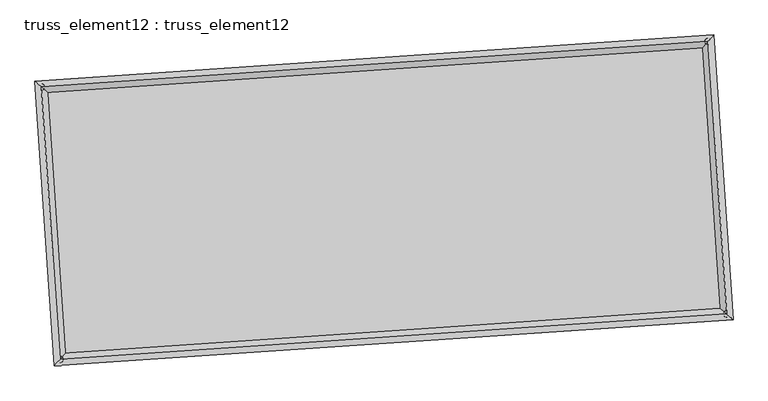
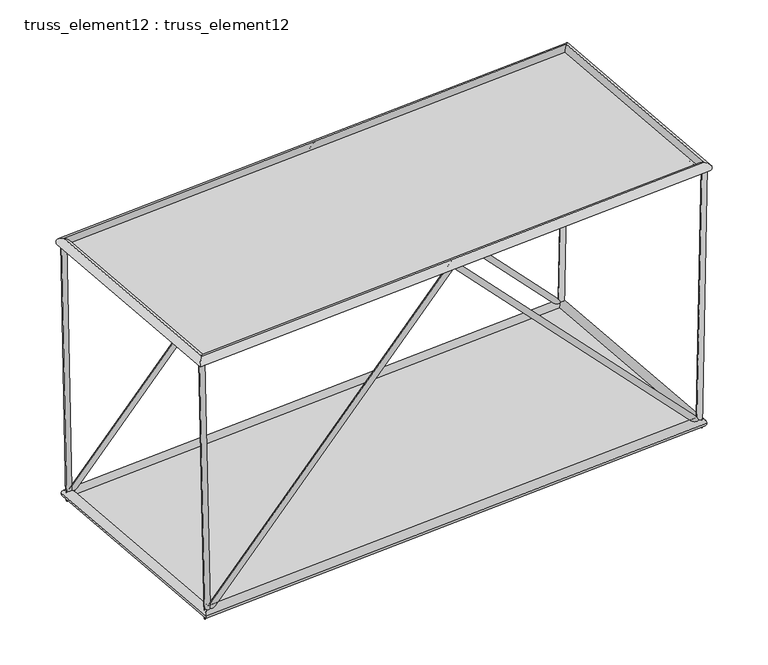
"""IFC4 building model written with IfcOpenShell, lengths in millimetres: plate geometry, truss_element12 : truss_element12."""

import ifcopenshell
import ifcopenshell.guid

model = None  # the IFC model being written
_history = None  # IfcOwnerHistory: only IFC2X3 demands one
_inside = {}  # id of a spatial element -> (the spatial element, [elements in it])
_under = {}  # id of a project, library or spatial element -> (it, [spatial elements below it])
_declared = {}  # id of a project -> (the project, [libraries it declares])
_typed = {}  # id of a type object -> (the type object, [elements of that type])
_made_of = {}  # id of a material, layer set ... -> (it, [elements and type objects made of it])


def new_model(schema):
    """Start an empty IFC model of exactly this schema.

    Asked for "IFC4X3", IfcOpenShell would pick the latest addendum, in which some entities
    have other attributes; the version numbers below select the first issue.
    IFC2X3 requires an IfcOwnerHistory on every rooted entity: one is made here for all.
    """
    global model, _history
    if schema == "IFC4X3":
        model = ifcopenshell.file(schema_version=(4, 3, 0, 0))
    else:
        model = ifcopenshell.file(schema=schema)
    _inside.clear()
    _under.clear()
    _declared.clear()
    _typed.clear()
    _made_of.clear()
    _history = None
    if model.schema == "IFC2X3":
        org = make("IfcOrganization", Name="unknown")
        user = make(
            "IfcPersonAndOrganization",
            ThePerson=make("IfcPerson", FamilyName="unknown"),
            TheOrganization=org,
        )
        app = make(
            "IfcApplication",
            ApplicationDeveloper=org,
            Version="unknown",
            ApplicationFullName="unknown",
            ApplicationIdentifier="unknown",
        )
        _history = make(
            "IfcOwnerHistory",
            OwningUser=user,
            OwningApplication=app,
            ChangeAction="ADDED",
            CreationDate=0,
        )
    return model


def make(cls, **values):
    """One entity of the class cls with the attributes given. An attribute that is None is left unset."""
    return model.create_entity(
        cls, **{name: value for name, value in values.items() if value is not None}
    )


def rooted(cls, **values):
    """An entity with a GlobalId (a new one), such as an element, a storey or a relation."""
    return make(cls, GlobalId=ifcopenshell.guid.new(), OwnerHistory=_history, **values)


def si_unit(unit_type, name, prefix=None):
    """IfcSIUnit, for example si_unit("LENGTHUNIT", "METRE", prefix="MILLI")."""
    return make("IfcSIUnit", UnitType=unit_type, Prefix=prefix, Name=name)


def assignment(units):
    """IfcUnitAssignment: the units of a project."""
    return None if units is None else make("IfcUnitAssignment", Units=units)


def point(xyz):
    """IfcCartesianPoint."""
    return None if xyz is None else make("IfcCartesianPoint", Coordinates=xyz)


def direction(xyz):
    """IfcDirection."""
    return None if xyz is None else make("IfcDirection", DirectionRatios=xyz)


def frame(location, z_axis=None, x_axis=None):
    """IfcAxis2Placement3D, a coordinate frame: its origin and axes. An axis left out is left unset."""
    return make(
        "IfcAxis2Placement3D",
        Location=point(location),
        Axis=direction(z_axis),
        RefDirection=direction(x_axis),
    )


def origin():
    """The frame at (0, 0, 0) with its axes left unset."""
    return frame((0.0, 0.0, 0.0))


def origin_with_axes():
    """The frame at (0, 0, 0) with the z axis (0, 0, 1) and the x axis (1, 0, 0) written out."""
    return frame((0.0, 0.0, 0.0), z_axis=(0.0, 0.0, 1.0), x_axis=(1.0, 0.0, 0.0))


def place(relative_to, where):
    """IfcLocalPlacement: puts the frame where relative to a parent placement (None: the world)."""
    return make(
        "IfcLocalPlacement", PlacementRelTo=relative_to, RelativePlacement=where
    )


def context(
    kind, dimensions, precision=None, world=None, true_north=None, identifier=None
):
    """IfcGeometricRepresentationContext, for example the 3D "Model" context."""
    return make(
        "IfcGeometricRepresentationContext",
        ContextIdentifier=identifier,
        ContextType=kind,
        CoordinateSpaceDimension=dimensions,
        Precision=precision,
        WorldCoordinateSystem=world,
        TrueNorth=true_north,
    )


def project(units=None, contexts=None):
    """IfcProject with its units and contexts."""
    return rooted(
        "IfcProject",
        Name="project",
        RepresentationContexts=contexts,
        UnitsInContext=assignment(units),
    )


def spatial(cls, under=None, at=None, **own):
    """A site, building, storey or space (cls), placed at a placement, below another one or the project."""
    s = rooted(cls, ObjectPlacement=at, **own)
    if under is not None:
        _under.setdefault(under.id(), (under, []))[1].append(s)
    return s


def polyline(points):
    """IfcPolyline through the points."""
    return make("IfcPolyline", Points=[point(p) for p in points])


def circle_curve(where, radius):
    """IfcCircle in the frame where."""
    return make("IfcCircle", Position=where, Radius=radius)


def ellipse_curve(where, semi_axis1, semi_axis2):
    """IfcEllipse in the frame where."""
    return make(
        "IfcEllipse", Position=where, SemiAxis1=semi_axis1, SemiAxis2=semi_axis2
    )


def outline(outer, holes=None, kind="AREA"):
    """IfcArbitraryClosedProfileDef: a profile drawn as a closed curve; with holes, ...WithVoids."""
    if holes is None:
        return make("IfcArbitraryClosedProfileDef", ProfileType=kind, OuterCurve=outer)
    return make(
        "IfcArbitraryProfileDefWithVoids",
        ProfileType=kind,
        OuterCurve=outer,
        InnerCurves=holes,
    )


def extrude(swept, where, along, depth):
    """IfcExtrudedAreaSolid: the profile swept, set in the frame where, extruded along a direction by depth."""
    return make(
        "IfcExtrudedAreaSolid",
        SweptArea=swept,
        Position=where,
        ExtrudedDirection=direction(along),
        Depth=depth,
    )


def shape(context_of_items, identifier, shape_type, items):
    """IfcShapeRepresentation: the items that make up one representation, for example the "Body"."""
    return make(
        "IfcShapeRepresentation",
        ContextOfItems=context_of_items,
        RepresentationIdentifier=identifier,
        RepresentationType=shape_type,
        Items=items,
    )


def source(mapping_origin, context_of_items, identifier, shape_type, items):
    """IfcRepresentationMap: a shape defined once, which mapped items show again and again."""
    return make(
        "IfcRepresentationMap",
        MappingOrigin=mapping_origin,
        MappedRepresentation=shape(context_of_items, identifier, shape_type, items),
    )


def transform(
    local_origin,
    x_axis=None,
    y_axis=None,
    z_axis=None,
    scale=None,
    scale2=None,
    scale3=None,
    uniform=True,
):
    """IfcCartesianTransformationOperator3D, or its non-uniform kind. x_axis, y_axis, z_axis: its Axis1, 2, 3."""
    if uniform:
        return make(
            "IfcCartesianTransformationOperator3D",
            Axis1=direction(x_axis),
            Axis2=direction(y_axis),
            LocalOrigin=point(local_origin),
            Scale=scale,
            Axis3=direction(z_axis),
        )
    return make(
        "IfcCartesianTransformationOperator3DnonUniform",
        Axis1=direction(x_axis),
        Axis2=direction(y_axis),
        LocalOrigin=point(local_origin),
        Scale=scale,
        Axis3=direction(z_axis),
        Scale2=scale2,
        Scale3=scale3,
    )


def mapped(mapping_source, mapping_target):
    """IfcMappedItem: shows the shape of a source again, moved by a transform."""
    return make(
        "IfcMappedItem", MappingSource=mapping_source, MappingTarget=mapping_target
    )


def made_of(thing, what):
    """Note that an element or type object is made of a material, layer set ...; save() writes the relation."""
    if what is not None:
        _made_of.setdefault(what.id(), (what, []))[1].append(thing)
    return thing


def element(
    cls,
    number,
    at=None,
    inside=None,
    cuts=None,
    type_object=None,
    material=None,
    context=None,
    identifier="Body",
    shape_type=None,
    held_by="IfcProductDefinitionShape",
    body=None,
    shapes=None,
    **own,
):
    """One element of the class cls, such as IfcWall. Its Tag is "e" and its number.

    at: its placement. inside: the storey or other place that contains it. cuts: it is an
    opening in that element (IfcRelVoidsElement). A single representation is given by context,
    identifier, shape_type and body (its items); several are given by shapes. held_by: the class
    of the entity that holds the representations. save() writes the other relations.
    """
    e = rooted(cls, Tag="e%d" % number, ObjectPlacement=at, **own)
    if body is not None:
        shapes = [shape(context, identifier, shape_type, body)]
    if shapes is not None:
        e.Representation = make(held_by, Representations=shapes)
    if inside is not None:
        _inside.setdefault(inside.id(), (inside, []))[1].append(e)
    if cuts is not None:
        rooted(
            "IfcRelVoidsElement", RelatingBuildingElement=cuts, RelatedOpeningElement=e
        )
    if type_object is not None:
        _typed.setdefault(type_object.id(), (type_object, []))[1].append(e)
    return made_of(e, material)


def aggregate(whole, parts):
    """IfcRelAggregates: a whole, such as a stair, and the parts it consists of."""
    return rooted("IfcRelAggregates", RelatingObject=whole, RelatedObjects=parts)


def save(model, path):
    """Write the relations noted so far, then the file.

    IfcRelAggregates (storeys below a building ...), IfcRelContainedInSpatialStructure (elements
    in a storey), IfcRelDefinesByType, IfcRelAssociatesMaterial and IfcRelDeclares: one each for
    every whole, place, type object, material and project.
    """
    for whole, parts in _under.values():
        aggregate(whole, parts)
    for where, things in _inside.values():
        rooted(
            "IfcRelContainedInSpatialStructure",
            RelatedElements=things,
            RelatingStructure=where,
        )
    for kind, things in _typed.values():
        rooted("IfcRelDefinesByType", RelatedObjects=things, RelatingType=kind)
    for what, things in _made_of.values():
        rooted("IfcRelAssociatesMaterial", RelatedObjects=things, RelatingMaterial=what)
    for by, libraries in _declared.values():
        rooted("IfcRelDeclares", RelatingContext=by, RelatedDefinitions=libraries)
    model.write(path)


def plane_surface(at):
    """IfcPlane: the flat surface through the origin of the frame at, square to its z axis."""
    return make("IfcPlane", Position=at)


def cylinder_surface(at, radius):
    """IfcCylindricalSurface: all points at the distance radius from the z axis of the frame at."""
    return make("IfcCylindricalSurface", Position=at, Radius=radius)


def advanced_brep(points, edges, surfaces, faces):
    """IfcAdvancedBrep: a solid bounded by faces that lie on surfaces and meet in shared edges.

    An edge is (start, end): straight between two places in points (the first is 0);
    or (start, end, curve); or (start, end, curve, False) where it runs against its curve.
    A face is (place in surfaces, loops), or (place, loops, False) where it looks against
    its surface's normal. A loop lists edges by number (the first is 1), with a minus sign
    where the edge is run from its end to its start. The first loop is the outer one.
    """
    corners = [point(p) for p in points]
    vertices = [make("IfcVertexPoint", VertexGeometry=c) for c in corners]
    made = []
    for start, end, *more in edges:
        made.append(
            make(
                "IfcEdgeCurve",
                EdgeStart=vertices[start],
                EdgeEnd=vertices[end],
                EdgeGeometry=more[0] if more else make("IfcPolyline", Points=[corners[start], corners[end]]),
                SameSense=more[1] if len(more) > 1 else True,
            )
        )
    hull = []
    for where, loops, *sense in faces:
        bounds = []
        for j, loop in enumerate(loops):
            ring = [make("IfcOrientedEdge", EdgeElement=made[abs(k) - 1], Orientation=k > 0) for k in loop]
            bounds.append(
                make(
                    "IfcFaceOuterBound" if j == 0 else "IfcFaceBound",
                    Bound=make("IfcEdgeLoop", EdgeList=ring),
                    Orientation=True,
                )
            )
        hull.append(make("IfcAdvancedFace", Bounds=bounds, FaceSurface=surfaces[where], SameSense=sense[0] if sense else True))
    return make("IfcAdvancedBrep", Outer=make("IfcClosedShell", CfsFaces=hull))


def truss_element12_truss_element12_b131e6b3(model_context):
    return source(origin(), model_context, "Body", "SolidModel", [
        advanced_brep(
        [(-3768.4426764, 2269.1666348, 4999.9589336), (-3867.5246147, 2255.8068381, 4997.8888311), (-3667.4480193, 2276.0530765, 121.5783447), (-3761.5388635, 2263.0336036, -121.5783447), (1063.0770133, 2598.6095961, 5071.0530229), (1063.5348076, 2592.0370354, 4926.8211016), (5794.8562778, 2921.251637, 121.5871066), (5889.9046992, 2921.1288515, -121.5871066), (5894.6060324, 2928.0531935, 4999.9725392), (5994.5849006, 2928.2665965, 4997.9279449)],
        [
            (0, 1, circle_curve(frame((-3817.9836456, 2262.4867364, 4998.9238824), z_axis=(-0.02069804082979307, -0.0014113207235644356, 0.9997847764792298), x_axis=(-0.1335984293387775, 0.9910346065567788, -0.0013668522459998886)), 50.0)),
            (1, 0, circle_curve(frame((-3817.9836456, 2262.4867364, 4998.9238824), z_axis=(-0.02069804082979307, -0.0014113207235644356, 0.9997847764792298), x_axis=(-0.1335984293387775, 0.9910346065567788, -0.0013668522459998886)), 50.0)),
            (0, 2),
            (2, 3, ellipse_curve(frame((-3714.4934414, 2269.54334, 0.0), z_axis=(-0.9295901312719013, -0.06338521734851928, 0.3631039824397008), x_axis=(0.3622628143287531, 0.024701324219198188, 0.9317486237910038)), 130.7681897, 50.0)),
            (3, 1),
            (3, 2, ellipse_curve(frame((-3714.4934414, 2269.54334, 0.0), z_axis=(-0.9295901312719013, -0.06338521734851928, 0.3631039824397008), x_axis=(0.3622628143287531, 0.024701324219198188, 0.9317486237910038)), 130.7681897, 50.0)),
            (2, 4),
            (4, 5, ellipse_curve(frame((1063.3059105, 2595.3233157, 4998.9370622), z_axis=(-0.9976833938584647, -0.06802823807757281, -6.665670624892205e-05), x_axis=(6.650228906150557e-05, 4.534538292236935e-06, -0.9999999977784416)), 72.2729929, 50.0)),
            (5, 3),
            (5, 4, ellipse_curve(frame((1063.3059105, 2595.3233157, 4998.9370622), z_axis=(-0.9976833938584647, -0.06802823807757281, -6.665670624892205e-05), x_axis=(6.650228906150557e-05, 4.534538292236935e-06, -0.9999999977784416)), 72.2729929, 50.0)),
            (4, 6),
            (6, 7, ellipse_curve(frame((5842.3804885, 2921.1902443, 0.0), z_axis=(-0.9295196526265941, -0.06338041167761001, -0.3632852031070254), x_axis=(-0.3624436151795683, -0.024713652341926975, 0.9316779814954775)), 130.7875297, 50.0)),
            (7, 5),
            (7, 6, ellipse_curve(frame((5842.3804885, 2921.1902443, 0.0), z_axis=(-0.9295196526265941, -0.06338041167761001, -0.3632852031070254), x_axis=(-0.3624436151795683, -0.024713652341926975, 0.9316779814954775)), 130.7875297, 50.0)),
            (8, 9, circle_curve(frame((5944.5954665, 2928.159895, 4998.950242), z_axis=(0.02044299559371984, 0.0013939301584341597, 0.9997900484050983), x_axis=(-0.0021620821975439704, 0.9999967514320084, -0.001350009629994563)), 50.0)),
            (9, 8, circle_curve(frame((5944.5954665, 2928.159895, 4998.950242), z_axis=(0.02044299559371984, 0.0013939301584341597, 0.9997900484050983), x_axis=(-0.0021620821975439704, 0.9999967514320084, -0.001350009629994563)), 50.0)),
            (6, 8),
            (9, 7),
        ],
        [
            plane_surface(frame((-3817.9836456, 2312.4866866, 4998.9944636), z_axis=(-0.02069804082979222, -0.0014113207235603269, 0.9997847764792298), x_axis=(0.999785772606216, -2.9217833220407372e-05, 0.020698020207497326))),
            cylinder_surface(frame((-3817.9836456, 2262.4867364, 4998.9238824), z_axis=(-0.02069804082979307, -0.0014113207235644356, 0.9997847764792298), x_axis=(-0.1335984293387775, 0.9910346065567788, -0.0013668522459998886)), 50.0),
            cylinder_surface(frame((-3714.4934414, 2269.54334, 0.0), z_axis=(-0.6901706602776504, -0.047060113740035145, -0.7221148145459193), x_axis=(-0.02041427160093359, 0.9987522040196589, -0.04557732419610876)), 50.0),
            cylinder_surface(frame((1063.3059105, 2595.3233157, 4998.9370622), z_axis=(-0.6902666987206849, -0.04706666223638937, 0.7220225854799648), x_axis=(-0.11534052405583756, 0.9922795437132268, -0.04558366635972915)), 50.0),
            plane_surface(frame((5944.5954665, 2878.1599436, 4999.0199531), z_axis=(0.020442995593722254, 0.0013939301584386188, 0.9997900484050981), x_axis=(0.9997910201292843, -2.850206444371398e-05, -0.020442975724616754))),
            cylinder_surface(frame((5842.3804885, 2921.1902443, 0.0), z_axis=(-0.020442995593719836, -0.0013939301584341595, -0.9997900484050981), x_axis=(-0.0021620821975439704, 0.9999967514320084, -0.001350009629994563)), 50.0),
        ],
        [
            (0, [[1, 2]]),
            (1, [[-1, 3, 4, 5]]),
            (1, [[-2, -5, 6, -3]]),
            (2, [[-4, 7, 8, 9]]),
            (2, [[-6, -9, 10, -7]]),
            (3, [[-8, 11, 12, 13]]),
            (3, [[-10, -13, 14, -11]]),
            (4, [[15, 16]]),
            (5, [[-12, 17, -16, 18]]),
            (5, [[-14, -18, -15, -17]]),
        ],
    ),
        advanced_brep(
        [(-3496.3297235, -1721.5669495, 4999.9589336), (-3595.4116618, -1734.9267462, 4997.8888311), (-3395.3350664, -1714.6805078, 121.5783447), (-3489.4259106, -1727.6999807, -121.5783447), (1335.1899662, -1392.1239882, 5071.0530229), (1335.6477605, -1398.6965489, 4926.8211016), (6066.9692307, -1069.4819473, 121.5871066), (6162.0176521, -1069.6047328, -121.5871066), (6166.7189853, -1062.6803908, 4999.9725392), (6266.6978535, -1062.4669878, 4997.9279449)],
        [
            (0, 1, circle_curve(frame((-3545.8706927, -1728.2468479, 4998.9238824), z_axis=(-0.02069804082979312, -0.001411320723564435, 0.9997847764792299), x_axis=(-0.1335984293387778, 0.9910346065567789, -0.001366852245999902)), 50.0)),
            (1, 0, circle_curve(frame((-3545.8706927, -1728.2468479, 4998.9238824), z_axis=(-0.02069804082979312, -0.001411320723564435, 0.9997847764792299), x_axis=(-0.1335984293387778, 0.9910346065567789, -0.001366852245999902)), 50.0)),
            (0, 2),
            (2, 3, ellipse_curve(frame((-3442.3804885, -1721.1902443, 0.0), z_axis=(-0.929590131271901, -0.06338521734851939, 0.36310398243970093), x_axis=(0.36226281432875324, 0.024701324219198247, 0.9317486237910038)), 130.7681897, 50.0)),
            (3, 1),
            (3, 2, ellipse_curve(frame((-3442.3804885, -1721.1902443, 0.0), z_axis=(-0.929590131271901, -0.06338521734851939, 0.36310398243970093), x_axis=(0.36226281432875324, 0.024701324219198247, 0.9317486237910038)), 130.7681897, 50.0)),
            (2, 4),
            (4, 5, ellipse_curve(frame((1335.4188634, -1395.4102686, 4998.9370622), z_axis=(-0.9976833938584647, -0.06802823807757304, -6.665670624852088e-05), x_axis=(6.650228906104429e-05, 4.5345382922849825e-06, -0.9999999977784416)), 72.2729929, 50.0)),
            (5, 3),
            (5, 4, ellipse_curve(frame((1335.4188634, -1395.4102686, 4998.9370622), z_axis=(-0.9976833938584647, -0.06802823807757304, -6.665670624852088e-05), x_axis=(6.650228906104429e-05, 4.5345382922849825e-06, -0.9999999977784416)), 72.2729929, 50.0)),
            (4, 6),
            (6, 7, ellipse_curve(frame((6114.4934414, -1069.54334, 0.0), z_axis=(-0.9295196526265943, -0.06338041167761027, -0.3632852031070244), x_axis=(-0.3624436151795674, -0.02471365234192704, 0.9316779814954779)), 130.7875297, 50.0)),
            (7, 5),
            (7, 6, ellipse_curve(frame((6114.4934414, -1069.54334, 0.0), z_axis=(-0.9295196526265943, -0.06338041167761027, -0.3632852031070244), x_axis=(-0.3624436151795674, -0.02471365234192704, 0.9316779814954779)), 130.7875297, 50.0)),
            (8, 9, circle_curve(frame((6216.7084194, -1062.5736893, 4998.950242), z_axis=(0.020442995593720842, 0.0013939301584342109, 0.9997900484050981), x_axis=(-0.002162082197543998, 0.9999967514320084, -0.0013500096299946115)), 50.0)),
            (9, 8, circle_curve(frame((6216.7084194, -1062.5736893, 4998.950242), z_axis=(0.020442995593720842, 0.0013939301584342109, 0.9997900484050981), x_axis=(-0.002162082197543998, 0.9999967514320084, -0.0013500096299946115)), 50.0)),
            (6, 8),
            (9, 7),
        ],
        [
            plane_surface(frame((-3545.8706927, -1678.2468977, 4998.9944636), z_axis=(-0.020698040829792222, -0.0014113207235603234, 0.9997847764792299), x_axis=(0.999785772606216, -2.9217833220407372e-05, 0.020698020207497326))),
            cylinder_surface(frame((-3545.8706927, -1728.2468479, 4998.9238824), z_axis=(-0.020698040829793124, -0.0014113207235644351, 0.9997847764792301), x_axis=(-0.1335984293387778, 0.9910346065567789, -0.001366852245999902)), 50.0),
            cylinder_surface(frame((-3442.3804885, -1721.1902443, 0.0), z_axis=(-0.6901706602776506, -0.047060113740035256, -0.7221148145459192), x_axis=(-0.020414271600933634, 0.9987522040196589, -0.04557732419610887)), 50.0),
            cylinder_surface(frame((1335.4188634, -1395.4102686, 4998.9370622), z_axis=(-0.6902666987206844, -0.04706666223638954, 0.7220225854799652), x_axis=(-0.115340524055838, 0.9922795437132268, -0.0455836663597292)), 50.0),
            plane_surface(frame((6216.7084194, -1112.5736407, 4999.0199531), z_axis=(0.020442995593722254, 0.0013939301584386132, 0.9997900484050981), x_axis=(0.9997910201292843, -2.8502064444602157e-05, -0.020442975724616754))),
            cylinder_surface(frame((6114.4934414, -1069.54334, 0.0), z_axis=(-0.020442995593720842, -0.0013939301584342109, -0.9997900484050981), x_axis=(-0.002162082197543998, 0.9999967514320084, -0.0013500096299946115)), 50.0),
        ],
        [
            (0, [[1, 2]]),
            (1, [[-1, 3, 4, 5]]),
            (1, [[-2, -5, 6, -3]]),
            (2, [[-4, 7, 8, 9]]),
            (2, [[-6, -9, 10, -7]]),
            (3, [[-8, 11, 12, 13]]),
            (3, [[-10, -13, 14, -11]]),
            (4, [[15, 16]]),
            (5, [[-12, 17, -16, 18]]),
            (5, [[-14, -18, -15, -17]]),
        ],
    ),
        advanced_brep(
        [(-3545.8638321, -1728.2392441, 4908.9238827), (-3545.8775532, -1728.2544517, 5088.9238821), (-3817.9914747, 2262.4933386, 5088.9238821), (-3817.9758164, 2262.4801343, 4908.9238827), (5944.6018432, 2928.1674658, 5088.9502418), (5944.5890897, 2928.1523242, 4908.9502423), (6216.7157648, -1062.5803244, 5088.9502418), (6216.701074, -1062.5670541, 4908.9502423)],
        [
            (0, 1, ellipse_curve(frame((-3545.8706927, -1728.2468479, 4998.9238824), z_axis=(-0.7535719234028934, 0.657365466278261, -1.9048135840263405e-06), x_axis=(-0.6573654662755266, -0.7535719234052785, -1.904813584026813e-06)), 127.2792206, 90.0)),
            (1, 2),
            (2, 3, ellipse_curve(frame((-3817.9836456, 2262.4867364, 4998.9238824), z_axis=(-0.6573654662755267, -0.7535719234052785, -1.904813584027251e-06), x_axis=(0.7535719234028933, -0.6573654662782611, 1.9048135840267782e-06)), 127.2792206, 90.0)),
            (3, 0),
            (1, 0, ellipse_curve(frame((-3545.8706927, -1728.2468479, 4998.9238824), z_axis=(-0.7535719234028934, 0.657365466278261, -1.9048135840263405e-06), x_axis=(-0.6573654662755266, -0.7535719234052785, -1.904813584026813e-06)), 127.2792206, 90.0)),
            (3, 2, ellipse_curve(frame((-3817.9836456, 2262.4867364, 4998.9238824), z_axis=(-0.6573654662755267, -0.7535719234052785, -1.904813584027251e-06), x_axis=(0.7535719234028933, -0.6573654662782611, 1.9048135840267782e-06)), 127.2792206, 90.0)),
            (2, 4),
            (4, 5, ellipse_curve(frame((5944.5954665, 2928.159895, 4998.950242), z_axis=(-0.753571923402893, 0.6573654662782614, -1.904813584027219e-06), x_axis=(-0.6573654662755272, -0.7535719234052781, -1.9048135840268106e-06)), 127.2792206, 90.0)),
            (5, 3),
            (5, 4, ellipse_curve(frame((5944.5954665, 2928.159895, 4998.950242), z_axis=(-0.753571923402893, 0.6573654662782614, -1.904813584027219e-06), x_axis=(-0.6573654662755272, -0.7535719234052781, -1.9048135840268106e-06)), 127.2792206, 90.0)),
            (4, 6),
            (6, 7, ellipse_curve(frame((6216.7084194, -1062.5736893, 4998.950242), z_axis=(0.6573654662755272, 0.7535719234052781, 1.9048135840263727e-06), x_axis=(-0.7535719234028929, 0.6573654662782614, -1.9048135840267807e-06)), 127.2792206, 90.0)),
            (7, 5),
            (7, 6, ellipse_curve(frame((6216.7084194, -1062.5736893, 4998.950242), z_axis=(0.6573654662755272, 0.7535719234052781, 1.9048135840263727e-06), x_axis=(-0.7535719234028929, 0.6573654662782614, -1.9048135840267807e-06)), 127.2792206, 90.0)),
            (6, 1),
            (0, 7),
        ],
        [
            cylinder_surface(frame((-3545.8706927, -1728.2468479, 4998.9238824), z_axis=(0.06802823822869399, -0.9976833960748771, 0.0), x_axis=(-0.9976833927370898, -0.06802823800110296, -8.179899131153941e-05)), 90.0),
            cylinder_surface(frame((-3817.9836456, 2262.4867364, 4998.9238824), z_axis=(-0.9976833960712572, -0.06802823822844672, -2.6938132043235077e-06), x_axis=(-0.06802823780324489, 0.9976833929678072, -7.910517811564465e-05)), 90.0),
            cylinder_surface(frame((5944.5954665, 2928.159895, 4998.950242), z_axis=(-0.068028238228693, 0.9976833960748774, 0.0), x_axis=(0.9976833931622919, 0.06802823803009488, -7.64113649197499e-05)), 90.0),
            cylinder_surface(frame((6216.7084194, -1062.5736893, 4998.950242), z_axis=(0.9976833960712573, 0.06802823822844663, 2.6938132043228885e-06), x_axis=(0.06802823822844663, -0.9976833929388144, -7.910517811564467e-05)), 90.0),
        ],
        [
            (0, [[1, 2, 3, 4]]),
            (0, [[5, -4, 6, -2]]),
            (1, [[-3, 7, 8, 9]]),
            (1, [[-6, -9, 10, -7]]),
            (2, [[-8, 11, 12, 13]]),
            (2, [[-10, -13, 14, -11]]),
            (3, [[-12, 15, -1, 16]]),
            (3, [[-14, -16, -5, -15]]),
        ],
    ),
        advanced_brep(
        [(-3358.7115243, -1625.2761972, 0.0), (-3526.0494527, -1817.1042913, 0.0), (-3810.4074885, 2353.2123043, 0.0), (-3618.5793943, 2185.8743758, 0.0), (5926.0494527, 3017.1042913, 0.0), (5758.7115243, 2825.2761972, 0.0), (6210.4074885, -1153.2123043, 0.0), (6018.5793943, -985.8743758, 0.0)],
        [
            (0, 1, ellipse_curve(frame((-3442.3804885, -1721.1902443, 0.0), z_axis=(-0.7535719234054582, 0.6573654662780803, 0.0), x_axis=(-0.6573654662780802, -0.7535719234054585, 0.0)), 127.2792206, 90.0)),
            (1, 2),
            (2, 3, ellipse_curve(frame((-3714.4934414, 2269.54334, 0.0), z_axis=(-0.6573654662780803, -0.7535719234054583, 0.0), x_axis=(0.7535719234054582, -0.6573654662780803, 0.0)), 127.2792206, 90.0)),
            (3, 0),
            (1, 0, ellipse_curve(frame((-3442.3804885, -1721.1902443, 0.0), z_axis=(-0.7535719234054582, 0.6573654662780803, 0.0), x_axis=(-0.6573654662780802, -0.7535719234054585, 0.0)), 127.2792206, 90.0)),
            (3, 2, ellipse_curve(frame((-3714.4934414, 2269.54334, 0.0), z_axis=(-0.6573654662780803, -0.7535719234054583, 0.0), x_axis=(0.7535719234054582, -0.6573654662780803, 0.0)), 127.2792206, 90.0)),
            (2, 4),
            (4, 5, ellipse_curve(frame((5842.3804885, 2921.1902443, 0.0), z_axis=(-0.753571923405458, 0.6573654662780808, 0.0), x_axis=(-0.6573654662780808, -0.7535719234054579, 0.0)), 127.2792206, 90.0)),
            (5, 3),
            (5, 4, ellipse_curve(frame((5842.3804885, 2921.1902443, 0.0), z_axis=(-0.753571923405458, 0.6573654662780808, 0.0), x_axis=(-0.6573654662780808, -0.7535719234054579, 0.0)), 127.2792206, 90.0)),
            (4, 6),
            (6, 7, ellipse_curve(frame((6114.4934414, -1069.54334, 0.0), z_axis=(0.6573654662780809, 0.7535719234054578, 0.0), x_axis=(-0.7535719234054576, 0.657365466278081, 0.0)), 127.2792206, 90.0)),
            (7, 5),
            (7, 6, ellipse_curve(frame((6114.4934414, -1069.54334, 0.0), z_axis=(0.6573654662780809, 0.7535719234054578, 0.0), x_axis=(-0.7535719234054576, 0.657365466278081, 0.0)), 127.2792206, 90.0)),
            (6, 1),
            (0, 7),
        ],
        [
            cylinder_surface(frame((-3442.3804885, -1721.1902443, 0.0), z_axis=(0.06802823822870205, -0.9976833960748765, 0.0), x_axis=(-0.9976833960748765, -0.06802823822870205, 0.0)), 90.0),
            cylinder_surface(frame((-3714.4934414, 2269.54334, 0.0), z_axis=(-0.9976833960748765, -0.06802823822870166, 0.0), x_axis=(-0.06802823822870166, 0.9976833960748765, 0.0)), 90.0),
            cylinder_surface(frame((5842.3804885, 2921.1902443, 0.0), z_axis=(-0.06802823822870079, 0.9976833960748767, 0.0), x_axis=(0.9976833960748767, 0.06802823822870079, 0.0)), 90.0),
            cylinder_surface(frame((6114.4934414, -1069.54334, 0.0), z_axis=(0.9976833960748767, 0.06802823822870135, 0.0), x_axis=(0.06802823822870135, -0.9976833960748767, 0.0)), 90.0),
        ],
        [
            (0, [[1, 2, 3, 4]]),
            (0, [[5, -4, 6, -2]]),
            (1, [[-3, 7, 8, 9]]),
            (1, [[-6, -9, 10, -7]]),
            (2, [[-8, 11, 12, 13]]),
            (2, [[-10, -13, 14, -11]]),
            (3, [[-12, 15, -1, 16]]),
            (3, [[-14, -16, -5, -15]]),
        ],
    ),
        extrude(outline(polyline([(-3442.3804885, -1721.1902443), (-3714.4934414, 2269.54334), (5842.3804885, 2921.1902443), (6114.4934414, -1069.54334), (-3442.3804885, -1721.1902443)])), origin_with_axes(), (0.0, 0.0, 1.0), 20.0),
        extrude(outline(polyline([(-2000.0, 4892.6238276), (2000.0, 4892.6238276), (1999.9999999, -4892.6238276), (-2000.0000001, -4892.6238276), (-2000.0, 4892.6238276)])), frame((1199.3623869, 599.9565236, 4998.9370622), z_axis=(-2.6875727060805124e-06, -1.8325536640732116e-07, 0.9999999999963718), x_axis=(-0.06802823822870185, 0.9976833960748765, 0.0)), (0.0, 0.0, 1.0), 20.0),
    ])


if __name__ == "__main__":
    model = new_model("IFC4")
    model_context = context("Model", 3, world=origin())
    ifc_project = project(units=[si_unit("LENGTHUNIT", "METRE", prefix="MILLI")], contexts=[model_context])
    site = spatial("IfcSite", under=ifc_project)
    building = spatial("IfcBuilding", under=site)
    placement = place(None, origin())
    truss_element12_truss_element12_shape = truss_element12_truss_element12_b131e6b3(model_context)
    element("IfcPlate", 1, ObjectType="truss_element12 : truss_element12", at=placement, inside=building, context=model_context, shape_type="MappedRepresentation", body=[
        mapped(truss_element12_truss_element12_shape, transform((0.0, 0.0, 0.0), x_axis=(1.0, 0.0, 0.0), y_axis=(0.0, 1.0, 0.0), z_axis=(0.0, 0.0, 1.0))),
    ])
    save(model, "model.ifc")

# Revit data of these elements
# Type "truss_element12 : truss_element12"
#   steellbar1 = 90 mm
#   steelbar2 = 50 mm
#   offset1 = 5000 mm
#   M = Default Roof
# Element 1 (IfcPlate, "truss_element12 : truss_element12")
#   Materials on its faces: "Default Roof"
# Materials
#   "Default Roof": class "Miscellaneous", colour RGB 0 127 0, transparency 0, Comments = "Rendering appearance not upgraded Rendering appearance not upgraded ", Cost = 0
